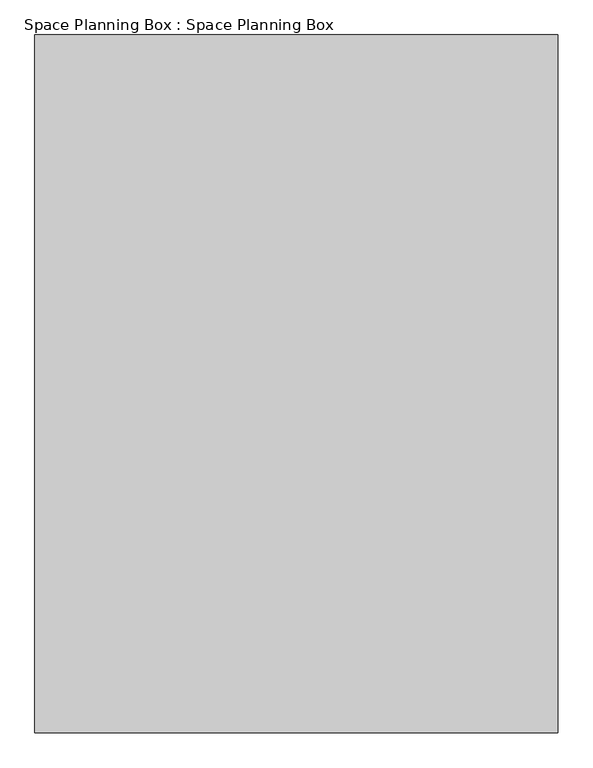
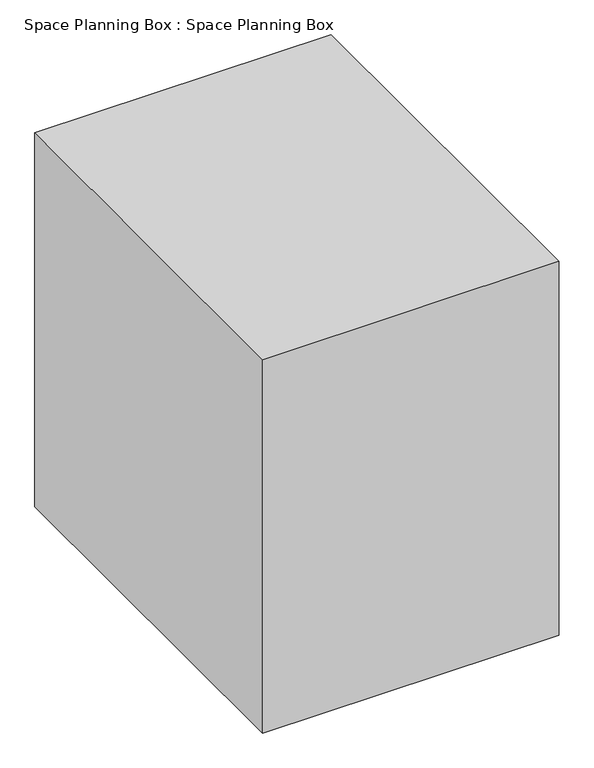
"""IFC4 building model written with IfcOpenShell, lengths in millimetres: proxy geometry, Space Planning Box : Space Planning Box."""

from ifc_helpers import new_model, si_unit, origin, origin_with_axes, place, context, project, spatial, polyline, outline, extrude, source, transform, mapped, element, save


def space_planning_box_space_planning_box_8af91fed(model_context):
    return source(origin(), model_context, "Body", "SweptSolid", [
        extrude(outline(polyline([(2250.0, 3000.0), (2250.0, -3000.0), (-2250.0, -3000.0), (-2250.0, 3000.0), (2250.0, 3000.0)])), origin_with_axes(), (0.0, 0.0, 1.0), 6000.0),
    ])


if __name__ == "__main__":
    model = new_model("IFC4")
    model_context = context("Model", 3, world=origin())
    ifc_project = project(units=[si_unit("LENGTHUNIT", "METRE", prefix="MILLI")], contexts=[model_context])
    site = spatial("IfcSite", under=ifc_project)
    building = spatial("IfcBuilding", under=site)
    placement = place(None, origin())
    space_planning_box_space_planning_box_shape = space_planning_box_space_planning_box_8af91fed(model_context)
    element("IfcBuildingElementProxy", 1, Name="Space Planning Box : Space Planning Box", ObjectType="Space Planning Box : Space Planning Box", at=placement, inside=building, context=model_context, shape_type="MappedRepresentation", body=[
        mapped(space_planning_box_space_planning_box_shape, transform((0.0, 0.0, 0.0), x_axis=(1.0, 0.0, 0.0), y_axis=(0.0, 1.0, 0.0), z_axis=(0.0, 0.0, 1.0))),
    ])
    save(model, "model.ifc")

# Revit data of these elements
# Type "Space Planning Box : Space Planning Box"
#   Type Comments = "..."
#   Room Name [instance default] = "?"
#   Assembly Code = "..."
#   Width [instance default] = 1524 mm
#   Program Area [instance default] = 0 m²
#   Length [instance default] = 1524 mm
#   Height [instance default] = 1524 mm
#   Area [instance default] = 2.32258 m²
#   Fill Color [instance default] = Cyan
#   Default Elevation = 0
# Element 1 (IfcBuildingElementProxy, "Space Planning Box : Space Planning Box")
#   Room Name = "Shift Office Room"
#   Width = 4500 mm
#   Program Area = 43.2 m²
#   Length = 6000 mm
#   Height = 6000 mm
#   Area = 27 m²
#   Fill Color = Lavender
#   Materials on its faces: "Lavender"
# Materials
#   "Cyan": class "Generic", colour RGB 0 255 255, transparency 0.2, Cost = 0
#   "Lavender": class "Generic", colour RGB 186 85 211, transparency 0.2, Cost = 0
